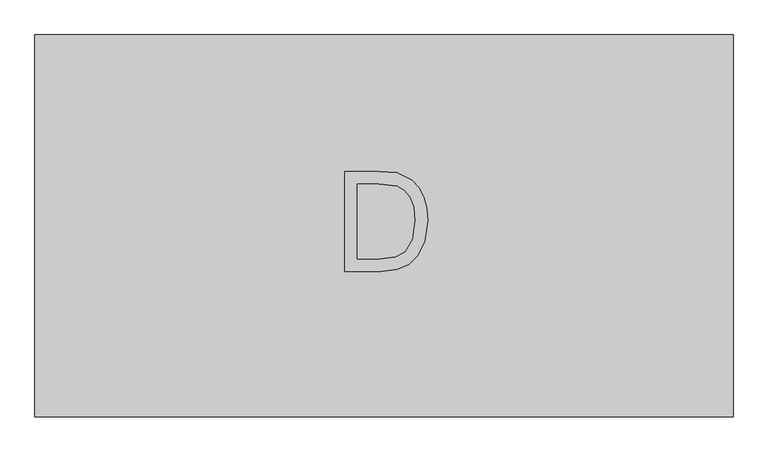
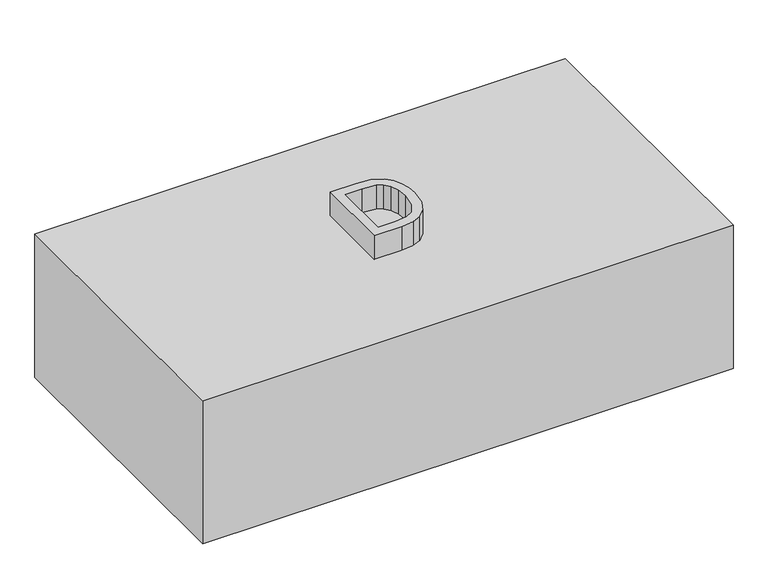
"""IFC4 building model written with IfcOpenShell, lengths in millimetres: proxy geometry, The Messy Family D : The Messy Family D."""

from ifc_helpers import new_model, si_unit, frame, origin, origin_with_axes, place, context, project, spatial, polyline, outline, extrude, source, transform, mapped, element, save


def generic_models_891ac883(model_context):
    return source(origin(), model_context, "Body", "SweptSolid", [
        extrude(outline(polyline([(541.9415527, 284.565081), (541.9415527, -299.634919), (-524.8584473, -299.634919), (-524.8584473, 284.565081), (541.9415527, 284.565081)])), origin_with_axes(), (0.0, 0.0, 1.0), 304.8),
        extrude(outline(polyline([(-51.7602961, -77.2556777), (-51.7602961, 75.839739), (1.0531375, 75.839739), (28.3755861, 73.6345072), (50.8764261, 62.6831016), (61.4634078, 51.0215367), (69.0041793, 36.5193341), (73.5174292, 19.45682), (75.0218459, 0.1143205), (70.9477735, -30.7776136), (60.4822665, -53.0728811), (46.5033393, -66.9583663), (28.2073904, -74.6393009), (3.5947606, -77.2556777), (-51.7602961, -77.2556777)]), holes=[polyline([(-32.623369, -58.1187506), (1.2400215, -58.1187506), (25.8713398, -55.3528666), (40.0745278, -47.5411132), (51.7174044, -28.5350049), (55.8849188, 0.413335), (53.8432105, 21.2695954), (47.7180856, 36.6688414), (38.6682253, 47.2464788), (27.8523107, 53.6379134), (0.7167462, 56.7028119), (-32.623369, 56.7028119), (-32.623369, -58.1187506)])]), frame((0.0, 0.0, 304.8), z_axis=(0.0, 0.0, 1.0), x_axis=(1.0, 0.0, 0.0)), (0.0, 0.0, 1.0), 50.8),
    ])


if __name__ == "__main__":
    model = new_model("IFC4")
    model_context = context("Model", 3, world=origin())
    ifc_project = project(units=[si_unit("LENGTHUNIT", "METRE", prefix="MILLI")], contexts=[model_context])
    site = spatial("IfcSite", under=ifc_project)
    building = spatial("IfcBuilding", under=site)
    placement = place(None, origin())
    generic_models_shape = generic_models_891ac883(model_context)
    element("IfcBuildingElementProxy", 1, Name="The Messy Family D : The Messy Family D", ObjectType="The Messy Family D : The Messy Family D", at=placement, inside=building, context=model_context, shape_type="MappedRepresentation", body=[
        mapped(generic_models_shape, transform((0.0, 0.0, 0.0), x_axis=(1.0, 0.0, 0.0), y_axis=(0.0, 1.0, 0.0), z_axis=(0.0, 0.0, 1.0))),
    ])
    save(model, "model.ifc")

# Revit data of these elements
# Type "The Messy Family D : The Messy Family D"
#   TBC-Parameter 2 = ""
#   TBC-Parameter 1 = ""
#   Other Company Parameter 2 = ""
#   Other Company Parameter 1 = ""
#   TBC-Parameter 3 = 2' - 0"
#   Other Company Parameter 3 = 1' - 0"
#   Default Elevation = 0
